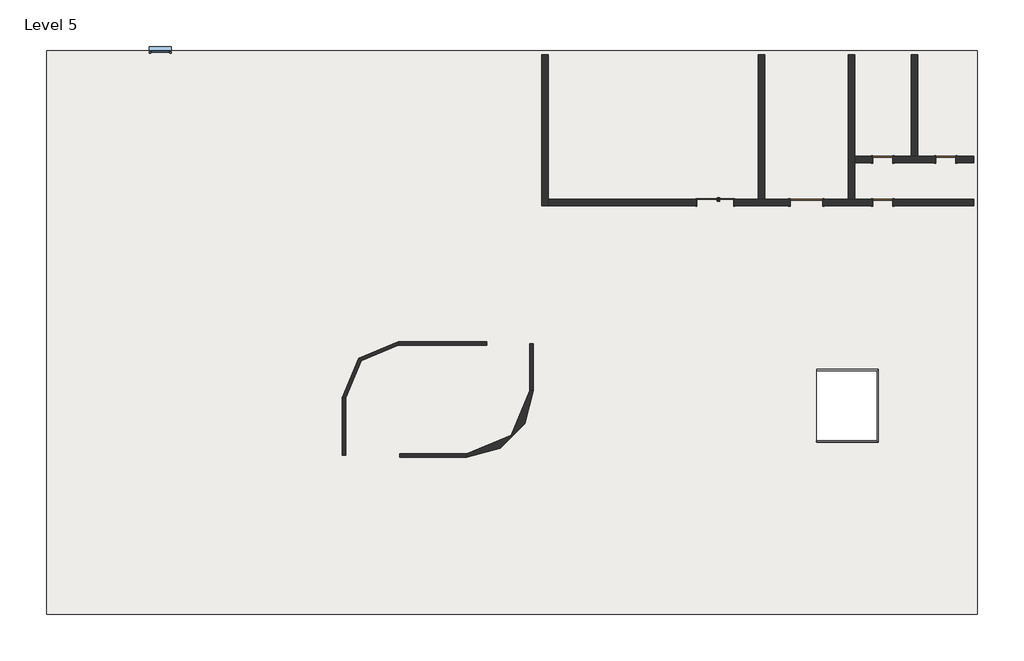
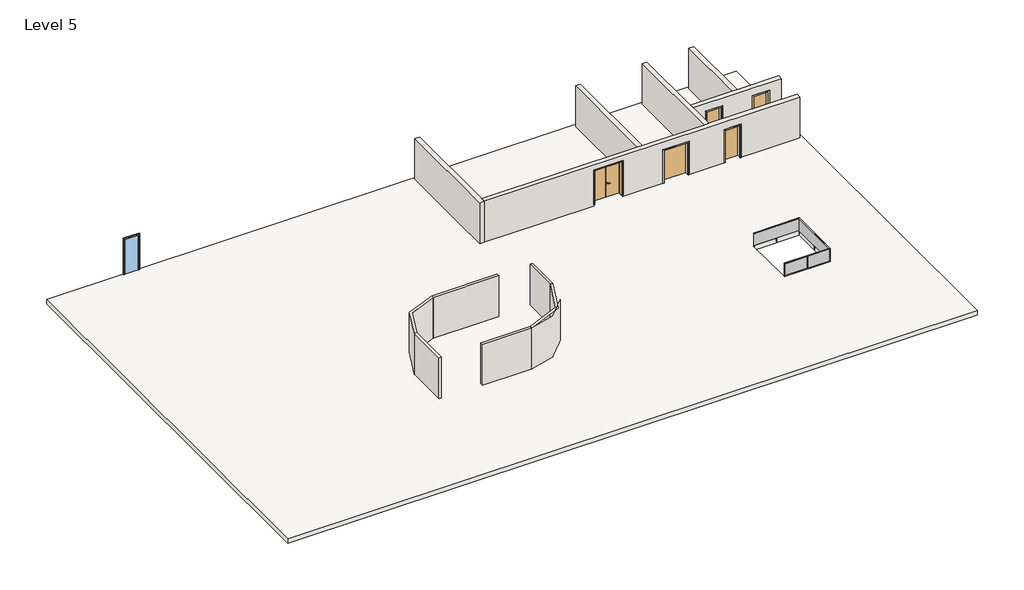
# One storey: 12 walls, 5 doors, 1 railing, 1 slab, 1 window.
"""IFC4 building model written with IfcOpenShell, lengths in millimetres."""

import ifcopenshell
import ifcopenshell.guid

model = None  # the IFC model being written
_history = None  # IfcOwnerHistory: only IFC2X3 demands one
_inside = {}  # id of a spatial element -> (the spatial element, [elements in it])
_under = {}  # id of a project, library or spatial element -> (it, [spatial elements below it])
_declared = {}  # id of a project -> (the project, [libraries it declares])
_typed = {}  # id of a type object -> (the type object, [elements of that type])
_made_of = {}  # id of a material, layer set ... -> (it, [elements and type objects made of it])


def new_model(schema):
    """Start an empty IFC model of exactly this schema.

    Asked for "IFC4X3", IfcOpenShell would pick the latest addendum, in which some entities
    have other attributes; the version numbers below select the first issue.
    IFC2X3 requires an IfcOwnerHistory on every rooted entity: one is made here for all.
    """
    global model, _history
    if schema == "IFC4X3":
        model = ifcopenshell.file(schema_version=(4, 3, 0, 0))
    else:
        model = ifcopenshell.file(schema=schema)
    _inside.clear()
    _under.clear()
    _declared.clear()
    _typed.clear()
    _made_of.clear()
    _history = None
    if model.schema == "IFC2X3":
        org = make("IfcOrganization", Name="unknown")
        user = make(
            "IfcPersonAndOrganization",
            ThePerson=make("IfcPerson", FamilyName="unknown"),
            TheOrganization=org,
        )
        app = make(
            "IfcApplication",
            ApplicationDeveloper=org,
            Version="unknown",
            ApplicationFullName="unknown",
            ApplicationIdentifier="unknown",
        )
        _history = make(
            "IfcOwnerHistory",
            OwningUser=user,
            OwningApplication=app,
            ChangeAction="ADDED",
            CreationDate=0,
        )
    return model


def make(cls, **values):
    """One entity of the class cls with the attributes given. An attribute that is None is left unset."""
    return model.create_entity(
        cls, **{name: value for name, value in values.items() if value is not None}
    )


def rooted(cls, **values):
    """An entity with a GlobalId (a new one), such as an element, a storey or a relation."""
    return make(cls, GlobalId=ifcopenshell.guid.new(), OwnerHistory=_history, **values)


def si_unit(unit_type, name, prefix=None):
    """IfcSIUnit, for example si_unit("LENGTHUNIT", "METRE", prefix="MILLI")."""
    return make("IfcSIUnit", UnitType=unit_type, Prefix=prefix, Name=name)


def assignment(units):
    """IfcUnitAssignment: the units of a project."""
    return None if units is None else make("IfcUnitAssignment", Units=units)


def point(xyz):
    """IfcCartesianPoint."""
    return None if xyz is None else make("IfcCartesianPoint", Coordinates=xyz)


def direction(xyz):
    """IfcDirection."""
    return None if xyz is None else make("IfcDirection", DirectionRatios=xyz)


def frame(location, z_axis=None, x_axis=None):
    """IfcAxis2Placement3D, a coordinate frame: its origin and axes. An axis left out is left unset."""
    return make(
        "IfcAxis2Placement3D",
        Location=point(location),
        Axis=direction(z_axis),
        RefDirection=direction(x_axis),
    )


def frame_2d(location, x_axis=None):
    """IfcAxis2Placement2D, a coordinate frame in the plane: its origin and x axis."""
    return make(
        "IfcAxis2Placement2D", Location=point(location), RefDirection=direction(x_axis)
    )


def origin():
    """The frame at (0, 0, 0) with its axes left unset."""
    return frame((0.0, 0.0, 0.0))


def origin_with_axes():
    """The frame at (0, 0, 0) with the z axis (0, 0, 1) and the x axis (1, 0, 0) written out."""
    return frame((0.0, 0.0, 0.0), z_axis=(0.0, 0.0, 1.0), x_axis=(1.0, 0.0, 0.0))


def place(relative_to, where):
    """IfcLocalPlacement: puts the frame where relative to a parent placement (None: the world)."""
    return make(
        "IfcLocalPlacement", PlacementRelTo=relative_to, RelativePlacement=where
    )


def context(
    kind, dimensions, precision=None, world=None, true_north=None, identifier=None
):
    """IfcGeometricRepresentationContext, for example the 3D "Model" context."""
    return make(
        "IfcGeometricRepresentationContext",
        ContextIdentifier=identifier,
        ContextType=kind,
        CoordinateSpaceDimension=dimensions,
        Precision=precision,
        WorldCoordinateSystem=world,
        TrueNorth=true_north,
    )


def project(units=None, contexts=None):
    """IfcProject with its units and contexts."""
    return rooted(
        "IfcProject",
        Name="project",
        RepresentationContexts=contexts,
        UnitsInContext=assignment(units),
    )


def spatial(cls, under=None, at=None, **own):
    """A site, building, storey or space (cls), placed at a placement, below another one or the project."""
    s = rooted(cls, ObjectPlacement=at, **own)
    if under is not None:
        _under.setdefault(under.id(), (under, []))[1].append(s)
    return s


def polyline(points):
    """IfcPolyline through the points."""
    return make("IfcPolyline", Points=[point(p) for p in points])


def circle_curve(where, radius):
    """IfcCircle in the frame where."""
    return make("IfcCircle", Position=where, Radius=radius)


def ellipse_curve(where, semi_axis1, semi_axis2):
    """IfcEllipse in the frame where."""
    return make(
        "IfcEllipse", Position=where, SemiAxis1=semi_axis1, SemiAxis2=semi_axis2
    )


def trimmed(basis, trim1, trim2, sense, master):
    """IfcTrimmedCurve: the piece of a basis curve between two trims."""
    return make(
        "IfcTrimmedCurve",
        BasisCurve=basis,
        Trim1=trim1,
        Trim2=trim2,
        SenseAgreement=sense,
        MasterRepresentation=master,
    )


def segment(curve, same_sense, transition):
    """IfcCompositeCurveSegment."""
    return make(
        "IfcCompositeCurveSegment",
        Transition=transition,
        SameSense=same_sense,
        ParentCurve=curve,
    )


def composite_curve(segments, self_intersect=None):
    """IfcCompositeCurve: segments joined end to end."""
    return make("IfcCompositeCurve", Segments=segments, SelfIntersect=self_intersect)


def outline(outer, holes=None, kind="AREA"):
    """IfcArbitraryClosedProfileDef: a profile drawn as a closed curve; with holes, ...WithVoids."""
    if holes is None:
        return make("IfcArbitraryClosedProfileDef", ProfileType=kind, OuterCurve=outer)
    return make(
        "IfcArbitraryProfileDefWithVoids",
        ProfileType=kind,
        OuterCurve=outer,
        InnerCurves=holes,
    )


def extrude(swept, where, along, depth):
    """IfcExtrudedAreaSolid: the profile swept, set in the frame where, extruded along a direction by depth."""
    return make(
        "IfcExtrudedAreaSolid",
        SweptArea=swept,
        Position=where,
        ExtrudedDirection=direction(along),
        Depth=depth,
    )


def faces_of(points, faces, orient=None, outer=None):
    """IfcFace entities. A face is a list of loops; a loop is a list of indices into points, from 0.

    orient and outer hold one flag for each loop. By default every Orientation is true, the
    first loop of a face is its IfcFaceOuterBound and the others are IfcFaceBound.
    """
    made = []
    for i, loops in enumerate(faces):
        bounds = []
        for j, loop in enumerate(loops):
            is_outer = j == 0 if outer is None else outer[i][j]
            bounds.append(
                make(
                    "IfcFaceOuterBound" if is_outer else "IfcFaceBound",
                    Bound=make("IfcPolyLoop", Polygon=[points[k] for k in loop]),
                    Orientation=True if orient is None else orient[i][j],
                )
            )
        made.append(make("IfcFace", Bounds=bounds))
    return made


def faceted_brep(points, faces, orient=None, outer=None, voids=None):
    """IfcFacetedBrep: a solid bounded by flat faces; with voids (closed shells), ...WithVoids."""
    shared = [point(p) for p in points]
    hull = make("IfcClosedShell", CfsFaces=faces_of(shared, faces, orient, outer))
    if voids is None:
        return make("IfcFacetedBrep", Outer=hull)
    return make(
        "IfcFacetedBrepWithVoids",
        Outer=hull,
        Voids=[
            make(cls, CfsFaces=faces_of(shared, fs, o, b)) for cls, fs, o, b in voids
        ],
    )


def shape(context_of_items, identifier, shape_type, items):
    """IfcShapeRepresentation: the items that make up one representation, for example the "Body"."""
    return make(
        "IfcShapeRepresentation",
        ContextOfItems=context_of_items,
        RepresentationIdentifier=identifier,
        RepresentationType=shape_type,
        Items=items,
    )


def source(mapping_origin, context_of_items, identifier, shape_type, items):
    """IfcRepresentationMap: a shape defined once, which mapped items show again and again."""
    return make(
        "IfcRepresentationMap",
        MappingOrigin=mapping_origin,
        MappedRepresentation=shape(context_of_items, identifier, shape_type, items),
    )


def transform(
    local_origin,
    x_axis=None,
    y_axis=None,
    z_axis=None,
    scale=None,
    scale2=None,
    scale3=None,
    uniform=True,
):
    """IfcCartesianTransformationOperator3D, or its non-uniform kind. x_axis, y_axis, z_axis: its Axis1, 2, 3."""
    if uniform:
        return make(
            "IfcCartesianTransformationOperator3D",
            Axis1=direction(x_axis),
            Axis2=direction(y_axis),
            LocalOrigin=point(local_origin),
            Scale=scale,
            Axis3=direction(z_axis),
        )
    return make(
        "IfcCartesianTransformationOperator3DnonUniform",
        Axis1=direction(x_axis),
        Axis2=direction(y_axis),
        LocalOrigin=point(local_origin),
        Scale=scale,
        Axis3=direction(z_axis),
        Scale2=scale2,
        Scale3=scale3,
    )


def mapped(mapping_source, mapping_target):
    """IfcMappedItem: shows the shape of a source again, moved by a transform."""
    return make(
        "IfcMappedItem", MappingSource=mapping_source, MappingTarget=mapping_target
    )


def made_of(thing, what):
    """Note that an element or type object is made of a material, layer set ...; save() writes the relation."""
    if what is not None:
        _made_of.setdefault(what.id(), (what, []))[1].append(thing)
    return thing


def element(
    cls,
    number,
    at=None,
    inside=None,
    cuts=None,
    type_object=None,
    material=None,
    context=None,
    identifier="Body",
    shape_type=None,
    held_by="IfcProductDefinitionShape",
    body=None,
    shapes=None,
    **own,
):
    """One element of the class cls, such as IfcWall. Its Tag is "e" and its number.

    at: its placement. inside: the storey or other place that contains it. cuts: it is an
    opening in that element (IfcRelVoidsElement). A single representation is given by context,
    identifier, shape_type and body (its items); several are given by shapes. held_by: the class
    of the entity that holds the representations. save() writes the other relations.
    """
    e = rooted(cls, Tag="e%d" % number, ObjectPlacement=at, **own)
    if body is not None:
        shapes = [shape(context, identifier, shape_type, body)]
    if shapes is not None:
        e.Representation = make(held_by, Representations=shapes)
    if inside is not None:
        _inside.setdefault(inside.id(), (inside, []))[1].append(e)
    if cuts is not None:
        rooted(
            "IfcRelVoidsElement", RelatingBuildingElement=cuts, RelatedOpeningElement=e
        )
    if type_object is not None:
        _typed.setdefault(type_object.id(), (type_object, []))[1].append(e)
    return made_of(e, material)


def aggregate(whole, parts):
    """IfcRelAggregates: a whole, such as a stair, and the parts it consists of."""
    return rooted("IfcRelAggregates", RelatingObject=whole, RelatedObjects=parts)


def save(model, path):
    """Write the relations noted so far, then the file.

    IfcRelAggregates (storeys below a building ...), IfcRelContainedInSpatialStructure (elements
    in a storey), IfcRelDefinesByType, IfcRelAssociatesMaterial and IfcRelDeclares: one each for
    every whole, place, type object, material and project.
    """
    for whole, parts in _under.values():
        aggregate(whole, parts)
    for where, things in _inside.values():
        rooted(
            "IfcRelContainedInSpatialStructure",
            RelatedElements=things,
            RelatingStructure=where,
        )
    for kind, things in _typed.values():
        rooted("IfcRelDefinesByType", RelatedObjects=things, RelatingType=kind)
    for what, things in _made_of.values():
        rooted("IfcRelAssociatesMaterial", RelatedObjects=things, RelatingMaterial=what)
    for by, libraries in _declared.values():
        rooted("IfcRelDeclares", RelatingContext=by, RelatedDefinitions=libraries)
    model.write(path)


def plane_surface(at):
    """IfcPlane: the flat surface through the origin of the frame at, square to its z axis."""
    return make("IfcPlane", Position=at)


def cylinder_surface(at, radius):
    """IfcCylindricalSurface: all points at the distance radius from the z axis of the frame at."""
    return make("IfcCylindricalSurface", Position=at, Radius=radius)


def advanced_brep(points, edges, surfaces, faces):
    """IfcAdvancedBrep: a solid bounded by faces that lie on surfaces and meet in shared edges.

    An edge is (start, end): straight between two places in points (the first is 0);
    or (start, end, curve); or (start, end, curve, False) where it runs against its curve.
    A face is (place in surfaces, loops), or (place, loops, False) where it looks against
    its surface's normal. A loop lists edges by number (the first is 1), with a minus sign
    where the edge is run from its end to its start. The first loop is the outer one.
    """
    corners = [point(p) for p in points]
    vertices = [make("IfcVertexPoint", VertexGeometry=c) for c in corners]
    made = []
    for start, end, *more in edges:
        made.append(
            make(
                "IfcEdgeCurve",
                EdgeStart=vertices[start],
                EdgeEnd=vertices[end],
                EdgeGeometry=more[0] if more else make("IfcPolyline", Points=[corners[start], corners[end]]),
                SameSense=more[1] if len(more) > 1 else True,
            )
        )
    hull = []
    for where, loops, *sense in faces:
        bounds = []
        for j, loop in enumerate(loops):
            ring = [make("IfcOrientedEdge", EdgeElement=made[abs(k) - 1], Orientation=k > 0) for k in loop]
            bounds.append(
                make(
                    "IfcFaceOuterBound" if j == 0 else "IfcFaceBound",
                    Bound=make("IfcEdgeLoop", EdgeList=ring),
                    Orientation=True,
                )
            )
        hull.append(make("IfcAdvancedFace", Bounds=bounds, FaceSurface=surfaces[where], SameSense=sense[0] if sense else True))
    return make("IfcAdvancedBrep", Outer=make("IfcClosedShell", CfsFaces=hull))


def door_double_flush_variable_door_double_flush_variable_ac6c3b87(model_context):
    return source(origin(), model_context, "Body", "SolidModel", [
        advanced_brep(
        [(90.0, 139.4346141, 1000.0), (110.0, 139.4346141, 1000.0), (90.0, 69.4346141, 1000.0), (110.0, 89.4346141, 1000.0), (220.0, 69.4346141, 1000.0), (220.0, 89.4346141, 1000.0)],
        [
            (0, 1, circle_curve(frame((100.0, 139.4346141, 1000.0), z_axis=(0.0, 1.0, 0.0), x_axis=(1.0, 0.0, 0.0)), 10.0)),
            (1, 0, circle_curve(frame((100.0, 139.4346141, 1000.0), z_axis=(0.0, 1.0, 0.0), x_axis=(1.0, 0.0, 0.0)), 10.0)),
            (0, 2),
            (2, 3, ellipse_curve(frame((100.0, 79.4346141, 1000.0), z_axis=(-0.7071067811865385, 0.7071067811865565, 0.0), x_axis=(0.7071067811865563, 0.7071067811865386, 0.0)), 14.1421356, 10.0)),
            (3, 1),
            (3, 2, ellipse_curve(frame((100.0, 79.4346141, 1000.0), z_axis=(-0.7071067811865385, 0.7071067811865565, 0.0), x_axis=(0.7071067811865563, 0.7071067811865386, 0.0)), 14.1421356, 10.0)),
            (4, 5, circle_curve(frame((220.0, 79.4346141, 1000.0), z_axis=(1.0, 0.0, 0.0), x_axis=(0.0, 1.0, 0.0)), 10.0)),
            (5, 4, circle_curve(frame((220.0, 79.4346141, 1000.0), z_axis=(1.0, 0.0, 0.0), x_axis=(0.0, 1.0, 0.0)), 10.0)),
            (2, 4),
            (5, 3),
        ],
        [
            plane_surface(frame((100.0, 139.4346141, -287.7526403), z_axis=(0.0, 1.0, 0.0), x_axis=(0.0, 0.0, 1.0))),
            cylinder_surface(frame((100.0, 139.4346141, 1000.0), z_axis=(0.0, 1.0, 0.0), x_axis=(1.0, 0.0, 0.0)), 10.0),
            plane_surface(frame((220.0, 79.4346141, -287.7526403), z_axis=(1.0, 0.0, 0.0), x_axis=(0.0, 0.0, 1.0))),
            cylinder_surface(frame((100.0, 79.4346141, 1000.0), z_axis=(-1.0, 0.0, 0.0), x_axis=(0.0, 1.0, 0.0)), 10.0),
        ],
        [
            (0, [[1, 2]]),
            (1, [[-1, 3, 4, 5]]),
            (1, [[-2, -5, 6, -3]]),
            (2, [[7, 8]]),
            (3, [[-4, 9, -8, 10]]),
            (3, [[-6, -10, -7, -9]]),
        ],
    ),
        advanced_brep(
        [(110.0, 199.4346141, 1000.0), (90.0, 199.4346141, 1000.0), (110.0, 229.4346141, 1000.0), (90.0, 249.4346141, 1000.0), (220.0, 229.4346141, 1000.0), (220.0, 249.4346141, 1000.0)],
        [
            (0, 1, circle_curve(frame((100.0, 199.4346141, 1000.0), z_axis=(0.0, -1.0, 0.0), x_axis=(-1.0, 0.0, 0.0)), 10.0)),
            (1, 0, circle_curve(frame((100.0, 199.4346141, 1000.0), z_axis=(0.0, -1.0, 0.0), x_axis=(-1.0, 0.0, 0.0)), 10.0)),
            (0, 2),
            (2, 3, ellipse_curve(frame((100.0, 239.4346141, 1000.0), z_axis=(-0.7071067811865475, -0.7071067811865475, 0.0), x_axis=(0.7071067811865474, -0.7071067811865476, 0.0)), 14.1421356, 10.0)),
            (3, 1),
            (3, 2, ellipse_curve(frame((100.0, 239.4346141, 1000.0), z_axis=(-0.7071067811865475, -0.7071067811865475, 0.0), x_axis=(0.7071067811865474, -0.7071067811865476, 0.0)), 14.1421356, 10.0)),
            (4, 5, circle_curve(frame((220.0, 239.4346141, 1000.0), z_axis=(1.0, 0.0, 0.0), x_axis=(0.0, 1.0, 0.0)), 10.0)),
            (5, 4, circle_curve(frame((220.0, 239.4346141, 1000.0), z_axis=(1.0, 0.0, 0.0), x_axis=(0.0, 1.0, 0.0)), 10.0)),
            (2, 4),
            (5, 3),
        ],
        [
            plane_surface(frame((100.0, 199.4346141, -287.7526403), z_axis=(0.0, -1.0, 0.0), x_axis=(0.0, 0.0, 1.0))),
            cylinder_surface(frame((100.0, 199.4346141, 1000.0), z_axis=(0.0, -1.0, 0.0), x_axis=(-1.0, 0.0, 0.0)), 10.0),
            plane_surface(frame((220.0, 239.4346141, -287.7526403), z_axis=(1.0, 0.0, 0.0), x_axis=(0.0, 0.0, 1.0))),
            cylinder_surface(frame((100.0, 239.4346141, 1000.0), z_axis=(-1.0, 0.0, 0.0), x_axis=(0.0, 1.0, 0.0)), 10.0),
        ],
        [
            (0, [[1, 2]]),
            (1, [[-1, 3, 4, 5]]),
            (1, [[-2, -5, 6, -3]]),
            (2, [[7, 8]]),
            (3, [[-4, 9, -8, 10]]),
            (3, [[-6, -10, -7, -9]]),
        ],
    ),
        extrude(outline(composite_curve([segment(trimmed(circle_curve(frame_2d((1000.0, 100.0)), 20.0), [point((1000.0, 80.0))], [point((1000.0, 120.0))], False, "CARTESIAN"), True, "CONTINUOUS"), segment(trimmed(circle_curve(frame_2d((1000.0, 100.0)), 20.0), [point((1000.0, 120.0))], [point((1000.0, 80.0))], False, "CARTESIAN"), True, "CONTINUOUS")], self_intersect=False)), frame((0.0, 129.4346141, 0.0), z_axis=(0.0, 1.0, 0.0), x_axis=(0.0, 0.0, 1.0)), (0.0, 0.0, 1.0), 10.0),
        extrude(outline(composite_curve([segment(trimmed(circle_curve(frame_2d((1000.0, 100.0)), 20.0), [point((1000.0, 80.0))], [point((1000.0, 120.0))], False, "CARTESIAN"), True, "CONTINUOUS"), segment(trimmed(circle_curve(frame_2d((1000.0, 100.0)), 20.0), [point((1000.0, 120.0))], [point((1000.0, 80.0))], False, "CARTESIAN"), True, "CONTINUOUS")], self_intersect=False)), frame((0.0, 189.4346141, 0.0), z_axis=(0.0, 1.0, 0.0), x_axis=(0.0, 0.0, 1.0)), (0.0, 0.0, 1.0), 10.0),
        extrude(outline(polyline([(0.0, 164.4346141), (-871.25, 164.4346141), (-871.25, 189.4346141), (0.0, 189.4346141), (0.0, 164.4346141)])), frame((0.0, 0.0, 100.0), z_axis=(0.0, 0.0, 1.0), x_axis=(1.0, 0.0, 0.0)), (0.0, 0.0, 1.0), 2250.0),
        extrude(outline(polyline([(871.25, 164.4346141), (0.0, 164.4346141), (0.0, 189.4346141), (871.25, 189.4346141), (871.25, 164.4346141)])), frame((0.0, 0.0, 100.0), z_axis=(0.0, 0.0, 1.0), x_axis=(1.0, 0.0, 0.0)), (0.0, 0.0, 1.0), 2250.0),
        faceted_brep([(905.75, -150.5653859, 100.0), (856.25, -150.5653859, 100.0), (856.25, 164.4346141, 100.0), (871.25, 164.4346141, 100.0), (871.25, 189.4346141, 100.0), (905.75, 189.4346141, 100.0), (905.75, 164.4346141, 100.0), (900.75, 164.4346141, 100.0), (900.75, 184.4346141, 100.0), (876.25, 184.4346141, 100.0), (876.25, 159.4346141, 100.0), (861.25, 159.4346141, 100.0), (861.25, -145.5653859, 100.0), (900.75, -145.5653859, 100.0), (900.75, -135.5653859, 100.0), (905.75, -135.5653859, 100.0), (905.75, -150.5653859, 2384.5), (-905.75, -150.5653859, 2384.5), (-905.75, -150.5653859, 100.0), (-856.25, -150.5653859, 100.0), (-856.25, -150.5653859, 2335.0), (856.25, -150.5653859, 2335.0), (856.25, 164.4346141, 2335.0), (-856.25, 164.4346141, 2335.0), (-856.25, 164.4346141, 100.0), (-871.25, 164.4346141, 100.0), (-871.25, 164.4346141, 2350.0), (871.25, 164.4346141, 2350.0), (871.25, 189.4346141, 2350.0), (-871.25, 189.4346141, 2350.0), (-871.25, 189.4346141, 100.0), (-905.75, 189.4346141, 100.0), (-905.75, 189.4346141, 2384.5), (905.75, 189.4346141, 2384.5), (905.75, 164.4346141, 2384.5), (-905.75, 164.4346141, 2384.5), (-905.75, 164.4346141, 100.0), (-900.75, 164.4346141, 100.0), (-900.75, 164.4346141, 2379.5), (900.75, 164.4346141, 2379.5), (900.75, 184.4346141, 2379.5), (-900.75, 184.4346141, 2379.5), (-900.75, 184.4346141, 100.0), (-876.25, 184.4346141, 100.0), (-876.25, 184.4346141, 2355.0), (876.25, 184.4346141, 2355.0), (876.25, 159.4346141, 2355.0), (-876.25, 159.4346141, 2355.0), (-876.25, 159.4346141, 100.0), (-861.25, 159.4346141, 100.0), (-861.25, 159.4346141, 2340.0), (861.25, 159.4346141, 2340.0), (861.25, -145.5653859, 2340.0), (-861.25, -145.5653859, 2340.0), (-861.25, -145.5653859, 100.0), (-900.75, -145.5653859, 100.0), (-900.75, -145.5653859, 2379.5), (900.75, -145.5653859, 2379.5), (900.75, -135.5653859, 2379.5), (-900.75, -135.5653859, 2379.5), (-900.75, -135.5653859, 100.0), (-905.75, -135.5653859, 100.0), (-905.75, -135.5653859, 2384.5), (905.75, -135.5653859, 2384.5)], [[[0, 1, 2, 3, 4, 5, 6, 7, 8, 9, 10, 11, 12, 13, 14, 15]], [[1, 0, 16, 17, 18, 19, 20, 21]], [[2, 1, 21, 22]], [[3, 2, 22, 23, 24, 25, 26, 27]], [[4, 3, 27, 28]], [[5, 4, 28, 29, 30, 31, 32, 33]], [[6, 5, 33, 34]], [[7, 6, 34, 35, 36, 37, 38, 39]], [[8, 7, 39, 40]], [[9, 8, 40, 41, 42, 43, 44, 45]], [[10, 9, 45, 46]], [[11, 10, 46, 47, 48, 49, 50, 51]], [[12, 11, 51, 52]], [[13, 12, 52, 53, 54, 55, 56, 57]], [[14, 13, 57, 58]], [[15, 14, 58, 59, 60, 61, 62, 63]], [[0, 15, 63, 16]], [[17, 62, 61, 18]], [[18, 61, 60, 55, 54, 49, 48, 43, 42, 37, 36, 31, 30, 25, 24, 19]], [[23, 20, 19, 24]], [[29, 26, 25, 30]], [[35, 32, 31, 36]], [[41, 38, 37, 42]], [[47, 44, 43, 48]], [[53, 50, 49, 54]], [[59, 56, 55, 60]], [[22, 21, 20, 23]], [[28, 27, 26, 29]], [[34, 33, 32, 35]], [[40, 39, 38, 41]], [[46, 45, 44, 47]], [[52, 51, 50, 53]], [[58, 57, 56, 59]], [[16, 63, 62, 17]]]),
    ])


def m_single_flush_0915_x_2134mm_1c84716f(model_context):
    return source(origin(), model_context, "Body", "SweptSolid", [
        extrude(outline(polyline([(2210.0, -533.5), (0.0, -533.5), (0.0, -457.5), (2134.0, -457.5), (2134.0, 457.5), (0.0, 457.5), (0.0, 533.5), (2210.0, 533.5), (2210.0, -533.5)])), frame((0.0, -175.0, 0.0), z_axis=(0.0, 1.0, 0.0), x_axis=(0.0, 0.0, 1.0)), (0.0, 0.0, 1.0), 25.0),
        extrude(outline(polyline([(2210.0, 533.5), (2210.0, -533.5), (0.0, -533.5), (0.0, -457.5), (2134.0, -457.5), (2134.0, 457.5), (0.0, 457.5), (0.0, 533.5), (2210.0, 533.5)])), frame((0.0, 150.0, 0.0), z_axis=(0.0, 1.0, 0.0), x_axis=(0.0, 0.0, 1.0)), (0.0, 0.0, 1.0), 25.0),
        extrude(outline(polyline([(457.5, -99.0), (457.5, -150.0), (-457.5, -150.0), (-457.5, -99.0), (457.5, -99.0)])), origin_with_axes(), (0.0, 0.0, 1.0), 2134.0),
    ])


def m_single_flush_1500_x_2134mm_2_edebd810(model_context):
    return source(origin(), model_context, "Body", "SweptSolid", [
        extrude(outline(polyline([(2210.0, -826.0), (0.0, -826.0), (0.0, -750.0), (2134.0, -750.0), (2134.0, 750.0), (0.0, 750.0), (0.0, 826.0), (2210.0, 826.0), (2210.0, -826.0)])), frame((0.0, -175.0, 0.0), z_axis=(0.0, 1.0, 0.0), x_axis=(0.0, 0.0, 1.0)), (0.0, 0.0, 1.0), 25.0),
        extrude(outline(polyline([(2210.0, 826.0), (2210.0, -826.0), (0.0, -826.0), (0.0, -750.0), (2134.0, -750.0), (2134.0, 750.0), (0.0, 750.0), (0.0, 826.0), (2210.0, 826.0)])), frame((0.0, 150.0, 0.0), z_axis=(0.0, 1.0, 0.0), x_axis=(0.0, 0.0, 1.0)), (0.0, 0.0, 1.0), 25.0),
        extrude(outline(polyline([(750.0, -99.0), (750.0, -150.0), (-750.0, -150.0), (-750.0, -99.0), (750.0, -99.0)])), origin_with_axes(), (0.0, 0.0, 1.0), 2134.0),
    ])


def glas_mpk_389492d2(model_context):
    return source(origin(), model_context, "Body", "SolidModel", [
        faceted_brep([(28820.4268037, 1294.9571597, 12843.2628643), (28820.4268037, 1244.9571597, 12843.2628643), (28820.4268037, 1244.9571597, 12856.7371357), (28820.4268037, 1294.9571597, 12856.7371357), (31660.4268037, 1294.9571597, 12843.2628643), (31610.4268037, 1244.9571597, 12843.2628643), (31610.4268037, 1244.9571597, 12856.7371357), (31660.4268037, 1294.9571597, 12856.7371357), (31660.4268037, -2045.7721864, 12843.2628643), (31610.4268037, -1995.7721864, 12843.2628643), (31610.4268037, -1995.7721864, 12856.7371357), (31660.4268037, -2045.7721864, 12856.7371357), (28820.4268037, -2045.7721864, 12843.2628643), (28820.4268037, -2045.7721864, 12856.7371357), (28820.4268037, -1995.7721864, 12856.7371357), (28820.4268037, -1995.7721864, 12843.2628643)], [[[0, 1, 2, 3]], [[1, 0, 4, 5]], [[2, 1, 5, 6]], [[3, 2, 6, 7]], [[0, 3, 7, 4]], [[5, 4, 8, 9]], [[6, 5, 9, 10]], [[7, 6, 10, 11]], [[4, 7, 11, 8]], [[12, 13, 14, 15]], [[9, 8, 12, 15]], [[10, 9, 15, 14]], [[11, 10, 14, 13]], [[8, 11, 13, 12]]]),
        faceted_brep([(28820.4268037, 1254.9571597, 12842.8769824), (28820.4268037, 1269.1492837, 12842.8769824), (28820.4268037, 1269.1492837, 12042.8769824), (28820.4268037, 1254.9571597, 12042.8769824), (31620.4268037, 1254.9571597, 12842.8769824), (31634.6189277, 1269.1492837, 12842.8769824), (31634.6189277, 1269.1492837, 12042.8769824), (31620.4268037, 1254.9571597, 12042.8769824), (31620.4268037, -2005.7721864, 12842.8769824), (31634.6189277, -2019.9643104, 12842.8769824), (31634.6189277, -2019.9643104, 12042.8769824), (31620.4268037, -2005.7721864, 12042.8769824), (28820.4268037, -2005.7721864, 12842.8769824), (28820.4268037, -2005.7721864, 12042.8769824), (28820.4268037, -2019.9643104, 12042.8769824), (28820.4268037, -2019.9643104, 12842.8769824)], [[[0, 1, 2, 3]], [[1, 0, 4, 5]], [[2, 1, 5, 6]], [[3, 2, 6, 7]], [[0, 3, 7, 4]], [[5, 4, 8, 9]], [[6, 5, 9, 10]], [[7, 6, 10, 11]], [[4, 7, 11, 8]], [[12, 13, 14, 15]], [[9, 8, 12, 15]], [[10, 9, 15, 14]], [[11, 10, 14, 13]], [[8, 11, 13, 12]]]),
        extrude(outline(polyline([(30251.6768037, -2020.7721864), (30251.6768037, -2045.7721864), (30226.6768037, -2045.7721864), (30226.6768037, -2020.7721864), (30251.6768037, -2020.7721864)])), frame((0.0, 0.0, 11800.0), z_axis=(0.0, 0.0, 1.0), x_axis=(1.0, 0.0, 0.0)), (0.0, 0.0, 1.0), 1043.2628643),
        extrude(outline(polyline([(31635.4268037, -362.9075133), (31660.4268037, -362.9075133), (31660.4268037, -387.9075133), (31635.4268037, -387.9075133), (31635.4268037, -362.9075133)])), frame((0.0, 0.0, 11800.0), z_axis=(0.0, 0.0, 1.0), x_axis=(1.0, 0.0, 0.0)), (0.0, 0.0, 1.0), 1043.2628643),
        extrude(outline(polyline([(30226.6768037, 1269.9571597), (30226.6768037, 1294.9571597), (30251.6768037, 1294.9571597), (30251.6768037, 1269.9571597), (30226.6768037, 1269.9571597)])), frame((0.0, 0.0, 11800.0), z_axis=(0.0, 0.0, 1.0), x_axis=(1.0, 0.0, 0.0)), (0.0, 0.0, 1.0), 1043.2628643),
        extrude(outline(polyline([(31635.4268037, -2030.7721864), (31660.4268037, -2030.7721864), (31660.4268037, -2055.7721864), (31635.4268037, -2055.7721864), (31635.4268037, -2030.7721864)])), frame((0.0, 0.0, 11800.0), z_axis=(0.0, 0.0, 1.0), x_axis=(1.0, 0.0, 0.0)), (0.0, 0.0, 1.0), 1043.2628643),
        extrude(outline(polyline([(31645.4268037, 1269.9571597), (31645.4268037, 1294.9571597), (31670.4268037, 1294.9571597), (31670.4268037, 1269.9571597), (31645.4268037, 1269.9571597)])), frame((0.0, 0.0, 11800.0), z_axis=(0.0, 0.0, 1.0), x_axis=(1.0, 0.0, 0.0)), (0.0, 0.0, 1.0), 1043.2628643),
        extrude(outline(polyline([(28832.9268037, -2020.7721864), (28832.9268037, -2045.7721864), (28807.9268037, -2045.7721864), (28807.9268037, -2020.7721864), (28832.9268037, -2020.7721864)])), frame((0.0, 0.0, 11800.0), z_axis=(0.0, 0.0, 1.0), x_axis=(1.0, 0.0, 0.0)), (0.0, 0.0, 1.0), 1043.2628643),
        extrude(outline(polyline([(28820.4268037, 1269.9571597), (28820.4268037, 1294.9571597), (28845.4268037, 1294.9571597), (28845.4268037, 1269.9571597), (28820.4268037, 1269.9571597)])), frame((0.0, 0.0, 11800.0), z_axis=(0.0, 0.0, 1.0), x_axis=(1.0, 0.0, 0.0)), (0.0, 0.0, 1.0), 1043.2628643),
    ])


def window_variable_standard_5cf830ff(model_context):
    return source(origin(), model_context, "Body", "SolidModel", [
        extrude(outline(polyline([(9000.0, 500.0), (9000.0, -500.0), (1000.0, -500.0), (1000.0, 500.0), (9000.0, 500.0)]), holes=[polyline([(8920.0, 440.0), (1080.0, 440.0), (1080.0, -440.0), (8920.0, -440.0), (8920.0, 440.0)])]), frame((0.0, 35.0, 0.0), z_axis=(0.0, 1.0, 0.0), x_axis=(0.0, 0.0, 1.0)), (0.0, 0.0, 1.0), 60.0),
        faceted_brep([(470.0, 35.0, 8950.0), (470.0, 5.0, 8950.0), (470.0, 5.0, 1050.0), (470.0, 35.0, 1050.0), (-470.0, 5.0, 8950.0), (-470.0, 5.0, 1050.0), (410.0, 5.0, 1110.0), (-410.0, 5.0, 1110.0), (-410.0, 5.0, 8890.0), (410.0, 5.0, 8890.0), (-470.0, 35.0, 1050.0), (-470.0, 35.0, 8950.0), (440.0, 35.0, 8920.0), (-440.0, 35.0, 8920.0), (-440.0, 35.0, 1080.0), (440.0, 35.0, 1080.0), (440.0, 65.0, 8920.0), (440.0, 65.0, 1080.0), (-440.0, 65.0, 1080.0), (-440.0, 65.0, 8920.0), (410.0, 65.0, 8890.0), (-410.0, 65.0, 8890.0), (-410.0, 65.0, 1110.0), (410.0, 65.0, 1110.0)], [[[0, 1, 2, 3]], [[1, 4, 5, 2], [6, 7, 8, 9]], [[3, 2, 5, 10]], [[3, 10, 11, 0], [12, 13, 14, 15]], [[16, 12, 15, 17]], [[17, 15, 14, 18]], [[17, 18, 19, 16], [20, 21, 22, 23]], [[9, 20, 23, 6]], [[6, 23, 22, 7]], [[10, 5, 4, 11]], [[18, 14, 13, 19]], [[7, 22, 21, 8]], [[11, 4, 1, 0]], [[19, 13, 12, 16]], [[8, 21, 20, 9]]]),
        extrude(outline(polyline([(-500.0, -205.0), (-500.0, 35.0), (500.0, 35.0), (500.0, -205.0), (-500.0, -205.0)])), frame((0.0, 0.0, 1005.0), z_axis=(0.0, 0.0, 1.0), x_axis=(1.0, 0.0, 0.0)), (0.0, 0.0, 1.0), 15.0),
        extrude(outline(polyline([(105.0221543, 1020.0), (205.0, 1000.0), (205.0, 990.0), (203.0, 990.0), (203.0, 998.3604634), (104.8240723, 1018.0), (95.0, 1018.0), (95.0, 1020.0), (105.0221543, 1020.0)])), frame((-500.0, 0.0, 0.0), z_axis=(1.0, 0.0, 0.0), x_axis=(0.0, 1.0, 0.0)), (0.0, 0.0, 1.0), 1000.0),
        extrude(outline(polyline([(410.0, 20.0), (-410.0, 20.0), (-410.0, 50.0), (410.0, 50.0), (410.0, 20.0)])), frame((0.0, 0.0, 1110.0), z_axis=(0.0, 0.0, 1.0), x_axis=(1.0, 0.0, 0.0)), (0.0, 0.0, 1.0), 7780.0),
    ])


model = new_model("IFC4")

# Units and contexts
model_context = context("Model", 3, world=origin())
ifc_project = project(units=[si_unit("LENGTHUNIT", "METRE", prefix="MILLI")], contexts=[model_context])

# Site, building, storey
site = spatial("IfcSite", under=ifc_project)
building = spatial("IfcBuilding", under=site)
storey = spatial("IfcBuildingStorey", under=building, Name="Level 5", Elevation=12000.0)

# Doors
placement = place(None, origin())
door_double_flush_variable_door_double_flush_variable_shape = door_double_flush_variable_door_double_flush_variable_ac6c3b87(model_context)
element("IfcDoor", 1, ObjectType="Door Double Flush - Variable : Door Double Flush - Variable", at=placement, inside=storey, context=model_context, shape_type="MappedRepresentation", body=[
    mapped(door_double_flush_variable_door_double_flush_variable_shape, transform((24136.7471367, 8984.3231089, 12000.0), x_axis=(1.0, 0.0, 0.0), y_axis=(0.0, 1.0, 0.0), z_axis=(0.0, 0.0, 1.0))),
])
m_single_flush_0915_x_2134mm_shape = m_single_flush_0915_x_2134mm_1c84716f(model_context)
element("IfcDoor", 2, ObjectType="M_Single-Flush : 0915 x 2134mm", at=placement, inside=storey, context=model_context, shape_type="MappedRepresentation", body=[
    mapped(m_single_flush_0915_x_2134mm_shape, transform((34787.1221367, 10998.757723, 12000.0), x_axis=(-1.0, 0.0, 0.0), y_axis=(0.0, -1.0, 0.0), z_axis=(0.0, 0.0, 1.0))),
])
element("IfcDoor", 3, ObjectType="M_Single-Flush : 0915 x 2134mm", at=placement, inside=storey, context=model_context, shape_type="MappedRepresentation", body=[
    mapped(m_single_flush_0915_x_2134mm_shape, transform((31874.3721367, 10998.757723, 12000.0), x_axis=(-1.0, 0.0, 0.0), y_axis=(0.0, -1.0, 0.0), z_axis=(0.0, 0.0, 1.0))),
])
element("IfcDoor", 4, ObjectType="M_Single-Flush : 0915 x 2134mm", at=placement, inside=storey, context=model_context, shape_type="MappedRepresentation", body=[
    mapped(m_single_flush_0915_x_2134mm_shape, transform((31874.3721367, 8998.757723, 12000.0), x_axis=(-1.0, 0.0, 0.0), y_axis=(0.0, -1.0, 0.0), z_axis=(0.0, 0.0, 1.0))),
])
m_single_flush_1500_x_2134mm_2_shape = m_single_flush_1500_x_2134mm_2_edebd810(model_context)
element("IfcDoor", 5, ObjectType="M_Single-Flush : 1500 x 2134mm 2", at=placement, inside=storey, context=model_context, shape_type="MappedRepresentation", body=[
    mapped(m_single_flush_1500_x_2134mm_2_shape, transform((28342.9971367, 8998.757723, 12000.0), x_axis=(-1.0, 0.0, 0.0), y_axis=(0.0, -1.0, 0.0), z_axis=(0.0, 0.0, 1.0))),
])

# Railing
glas_mpk_shape = glas_mpk_389492d2(model_context)
element("IfcRailing", 6, ObjectType="Glas - MPK", at=placement, inside=storey, context=model_context, shape_type="MappedRepresentation", body=[
    mapped(glas_mpk_shape, transform((0.0, 0.0, 0.0), x_axis=(1.0, 0.0, 0.0), y_axis=(0.0, 1.0, 0.0), z_axis=(0.0, 0.0, 1.0))),
])

# Slab
element("IfcSlab", 7, ObjectType="Generic 300mm", at=placement, inside=storey, context=model_context, shape_type="SweptSolid", body=[
    extrude(outline(polyline([(-6732.0028633, 15998.757723), (36243.4971367, 15998.757723), (36243.4971367, -10001.242277), (-6732.0028633, -10001.242277), (-6732.0028633, 15998.757723)]), holes=[polyline([(31663.0737371, 1305.1195288), (28813.0737371, 1305.1195288), (28813.0737371, -2055.6098174), (31663.0737371, -2055.6098174), (31663.0737371, 1305.1195288)])]), frame((0.0, 0.0, 11700.0), z_axis=(0.0, 0.0, 1.0), x_axis=(1.0, 0.0, 0.0)), (0.0, 0.0, 1.0), 300.0),
])

# Walls
element("IfcWall", 8, ObjectType="Generic - 300mm", at=placement, inside=storey, context=model_context, shape_type="Brep", body=[
    faceted_brep([(16117.9971367, 15823.757723, 12000.0), (16117.9971367, 8848.757723, 12000.0), (16117.9971367, 8848.757723, 14700.0), (16117.9971367, 15823.757723, 14700.0), (16417.9971367, 15823.757723, 12000.0), (16417.9971367, 15823.757723, 14700.0), (16417.9971367, 9148.757723, 14700.0), (16417.9971367, 8848.757723, 14700.0), (16417.9971367, 8848.757723, 12000.0), (16417.9971367, 9148.757723, 12000.0)], [[[0, 1, 2, 3]], [[4, 5, 6, 7, 8, 9]], [[1, 0, 4, 9, 8]], [[3, 2, 7, 6, 5]], [[2, 1, 8, 7]], [[0, 3, 5, 4]]]),
])
element("IfcWall", 9, ObjectType="Generic - 300mm", at=placement, inside=storey, context=model_context, shape_type="SweptSolid", body=[
    extrude(outline(polyline([(26117.9971367, 9148.757723), (26117.9971367, 15823.757723), (26417.9971367, 15823.757723), (26417.9971367, 9148.757723), (26117.9971367, 9148.757723)])), frame((0.0, 0.0, 12000.0), z_axis=(0.0, 0.0, 1.0), x_axis=(1.0, 0.0, 0.0)), (0.0, 0.0, 1.0), 2700.0),
])
element("IfcWall", 10, ObjectType="Generic - 300mm", at=placement, inside=storey, context=model_context, shape_type="Brep", body=[
    faceted_brep([(30267.9971367, 15823.757723, 12000.0), (30267.9971367, 9148.757723, 12000.0), (30267.9971367, 9148.757723, 14700.0), (30267.9971367, 15823.757723, 14700.0), (30567.9971367, 15823.757723, 12000.0), (30567.9971367, 15823.757723, 14700.0), (30567.9971367, 11148.757723, 14700.0), (30567.9971367, 10848.757723, 14700.0), (30567.9971367, 9148.757723, 14700.0), (30567.9971367, 9148.757723, 12000.0), (30567.9971367, 10848.757723, 12000.0), (30567.9971367, 11148.757723, 12000.0)], [[[0, 1, 2, 3]], [[4, 5, 6, 7, 8, 9, 10, 11]], [[1, 0, 4, 11, 10, 9]], [[3, 2, 8, 7, 6, 5]], [[2, 1, 9, 8]], [[0, 3, 5, 4]]]),
])
element("IfcWall", 11, ObjectType="Generic - 300mm", at=placement, inside=storey, context=model_context, shape_type="SweptSolid", body=[
    extrude(outline(polyline([(33180.7471367, 11148.757723), (33180.7471367, 15823.757723), (33480.7471367, 15823.757723), (33480.7471367, 11148.757723), (33180.7471367, 11148.757723)])), frame((0.0, 0.0, 12000.0), z_axis=(0.0, 0.0, 1.0), x_axis=(1.0, 0.0, 0.0)), (0.0, 0.0, 1.0), 2700.0),
])
element("IfcWall", 12, ObjectType="Generic - 300mm", at=placement, inside=storey, context=model_context, shape_type="Brep", body=[
    faceted_brep([(16417.9971367, 9148.757723, 14700.0), (26117.9971367, 9148.757723, 14700.0), (26417.9971367, 9148.757723, 14700.0), (30267.9971367, 9148.757723, 14700.0), (30567.9971367, 9148.757723, 14700.0), (36068.4971367, 9148.757723, 14700.0), (36068.4971367, 9148.757723, 12000.0), (32331.8721367, 9148.757723, 12000.0), (32331.8721367, 9148.757723, 14134.0), (31416.8721367, 9148.757723, 14134.0), (31416.8721367, 9148.757723, 12000.0), (30567.9971367, 9148.757723, 12000.0), (30267.9971367, 9148.757723, 12000.0), (29092.9971367, 9148.757723, 12000.0), (29092.9971367, 9148.757723, 14134.0), (27592.9971367, 9148.757723, 14134.0), (27592.9971367, 9148.757723, 12000.0), (26417.9971367, 9148.757723, 12000.0), (26117.9971367, 9148.757723, 12000.0), (25017.9971367, 9148.757723, 12000.0), (25017.9971367, 9148.757723, 14360.0), (23255.4971367, 9148.757723, 14360.0), (23255.4971367, 9148.757723, 12000.0), (16417.9971367, 9148.757723, 12000.0), (36068.4971367, 8848.757723, 14700.0), (16417.9971367, 8848.757723, 14700.0), (16417.9971367, 8848.757723, 12000.0), (23255.4971367, 8848.757723, 12000.0), (23255.4971367, 8848.757723, 14360.0), (25017.9971367, 8848.757723, 14360.0), (25017.9971367, 8848.757723, 12000.0), (27592.9971367, 8848.757723, 12000.0), (27592.9971367, 8848.757723, 14134.0), (29092.9971367, 8848.757723, 14134.0), (29092.9971367, 8848.757723, 12000.0), (31416.8721367, 8848.757723, 12000.0), (31416.8721367, 8848.757723, 14134.0), (32331.8721367, 8848.757723, 14134.0), (32331.8721367, 8848.757723, 12000.0), (36068.4971367, 8848.757723, 12000.0)], [[[0, 1, 2, 3, 4, 5, 6, 7, 8, 9, 10, 11, 12, 13, 14, 15, 16, 17, 18, 19, 20, 21, 22, 23]], [[24, 25, 26, 27, 28, 29, 30, 31, 32, 33, 34, 35, 36, 37, 38, 39]], [[26, 23, 22, 27]], [[10, 35, 34, 13, 12, 11]], [[38, 7, 6, 39]], [[16, 31, 30, 19, 18, 17]], [[5, 4, 3, 2, 1, 0, 25, 24]], [[0, 23, 26, 25]], [[36, 35, 10, 9]], [[37, 36, 9, 8]], [[38, 37, 8, 7]], [[32, 31, 16, 15]], [[33, 32, 15, 14]], [[34, 33, 14, 13]], [[29, 20, 19, 30]], [[20, 29, 28, 21]], [[21, 28, 27, 22]], [[6, 5, 24, 39]]]),
])
element("IfcWall", 13, ObjectType="Generic - 300mm", at=placement, inside=storey, context=model_context, shape_type="Brep", body=[
    faceted_brep([(31416.8721367, 11148.757723, 14134.0), (31416.8721367, 11148.757723, 12000.0), (30567.9971367, 11148.757723, 12000.0), (30567.9971367, 11148.757723, 14700.0), (33180.7471367, 11148.757723, 14700.0), (33480.7471367, 11148.757723, 14700.0), (36068.4971367, 11148.757723, 14700.0), (36068.4971367, 11148.757723, 12000.0), (35244.6221367, 11148.757723, 12000.0), (35244.6221367, 11148.757723, 14134.0), (34329.6221367, 11148.757723, 14134.0), (34329.6221367, 11148.757723, 12000.0), (33480.7471367, 11148.757723, 12000.0), (33180.7471367, 11148.757723, 12000.0), (32331.8721367, 11148.757723, 12000.0), (32331.8721367, 11148.757723, 14134.0), (30567.9971367, 10848.757723, 12000.0), (31416.8721367, 10848.757723, 12000.0), (31416.8721367, 10848.757723, 14134.0), (32331.8721367, 10848.757723, 14134.0), (32331.8721367, 10848.757723, 12000.0), (34329.6221367, 10848.757723, 12000.0), (34329.6221367, 10848.757723, 14134.0), (35244.6221367, 10848.757723, 14134.0), (35244.6221367, 10848.757723, 12000.0), (36068.4971367, 10848.757723, 12000.0), (36068.4971367, 10848.757723, 14700.0), (30567.9971367, 10848.757723, 14700.0)], [[[0, 1, 2, 3, 4, 5, 6, 7, 8, 9, 10, 11, 12, 13, 14, 15]], [[16, 17, 18, 19, 20, 21, 22, 23, 24, 25, 26, 27]], [[8, 7, 25, 24]], [[2, 1, 17, 16]], [[14, 13, 12, 11, 21, 20]], [[6, 5, 4, 3, 27, 26]], [[3, 2, 16, 27]], [[22, 21, 11, 10]], [[23, 22, 10, 9]], [[24, 23, 9, 8]], [[18, 17, 1, 0]], [[19, 18, 0, 15]], [[20, 19, 15, 14]], [[7, 6, 26, 25]]]),
])
element("IfcWall", 14, ObjectType="Interior - Blockwork 140", at=placement, inside=storey, context=model_context, shape_type="SweptSolid", body=[
    extrude(outline(polyline([(13583.5160614, 2407.0363043), (9501.5160614, 2407.0363043), (9501.5160614, 2571.0363043), (13583.5160614, 2571.0363043), (13583.5160614, 2407.0363043)])), frame((0.0, 0.0, 12000.0), z_axis=(0.0, 0.0, 1.0), x_axis=(1.0, 0.0, 0.0)), (0.0, 0.0, 1.0), 2700.0),
])
element("IfcWall", 15, ObjectType="Interior - Blockwork 140", at=placement, inside=storey, context=model_context, shape_type="SweptSolid", body=[
    extrude(outline(polyline([(7083.5160614, -10.9636957), (7083.5160614, -2674.9636957), (6919.5160614, -2674.9636957), (6919.5160614, -10.9636957), (7083.5160614, -10.9636957)])), frame((0.0, 0.0, 12000.0), z_axis=(0.0, 0.0, 1.0), x_axis=(1.0, 0.0, 0.0)), (0.0, 0.0, 1.0), 2700.0),
])
element("IfcWall", 16, ObjectType="Interior - Blockwork 140", at=placement, inside=storey, context=model_context, shape_type="SweptSolid", body=[
    extrude(outline(polyline([(9583.5160614, -2592.9636957), (12665.5160614, -2592.9636957), (12665.5160614, -2756.9636957), (9583.5160614, -2756.9636957), (9583.5160614, -2592.9636957)])), frame((0.0, 0.0, 12000.0), z_axis=(0.0, 0.0, 1.0), x_axis=(1.0, 0.0, 0.0)), (0.0, 0.0, 1.0), 2700.0),
])
element("IfcWall", 17, ObjectType="Interior - Blockwork 140", at=placement, inside=storey, context=model_context, shape_type="SweptSolid", body=[
    extrude(outline(polyline([(15583.5160614, 325.0363043), (15583.5160614, 2489.0363043), (15747.5160614, 2489.0363043), (15747.5160614, 325.0363043), (15583.5160614, 325.0363043)])), frame((0.0, 0.0, 12000.0), z_axis=(0.0, 0.0, 1.0), x_axis=(1.0, 0.0, 0.0)), (0.0, 0.0, 1.0), 2700.0),
])
element("IfcWall", 18, ObjectType="Interior - Blockwork 140", at=placement, inside=storey, context=model_context, shape_type="SweptSolid", body=[
    extrude(outline(composite_curve([segment(polyline([(7083.5160614, -10.9636957), (6919.5160614, -10.9636957)]), True, "CONTINUOUS"), segment(trimmed(circle_curve(frame_2d((9501.5160614, -10.9636957)), 2582.0), [point((6919.5160614, -10.9636957))], [point((9501.5160614, 2571.0363043))], False, "CARTESIAN"), True, "CONTINUOUS"), segment(polyline([(9501.5160614, 2571.0363043), (9501.5160614, 2407.0363043)]), True, "CONTINUOUS"), segment(trimmed(circle_curve(frame_2d((9501.5160614, -10.9636957)), 2418.0), [point((9501.5160614, 2407.0363043))], [point((7083.5160614, -10.9636957))], True, "CARTESIAN"), True, "CONTINUOUS")], self_intersect=False)), frame((0.0, 0.0, 12000.0), z_axis=(0.0, 0.0, 1.0), x_axis=(1.0, 0.0, 0.0)), (0.0, 0.0, 1.0), 2700.0),
])
element("IfcWall", 19, ObjectType="Interior - Blockwork 140", at=placement, inside=storey, context=model_context, shape_type="SweptSolid", body=[
    extrude(outline(composite_curve([segment(polyline([(15583.5160614, 325.0363043), (15747.5160614, 325.0363043)]), True, "CONTINUOUS"), segment(trimmed(circle_curve(frame_2d((12665.5160614, 325.0363043)), 3082.0), [point((15747.5160614, 325.0363043))], [point((12665.5160614, -2756.9636957))], False, "CARTESIAN"), True, "CONTINUOUS"), segment(polyline([(12665.5160614, -2756.9636957), (12665.5160614, -2592.9636957)]), True, "CONTINUOUS"), segment(trimmed(circle_curve(frame_2d((12665.5160614, 325.0363043)), 2918.0), [point((12665.5160614, -2592.9636957))], [point((15583.5160614, 325.0363043))], True, "CARTESIAN"), True, "CONTINUOUS")], self_intersect=False)), frame((0.0, 0.0, 12000.0), z_axis=(0.0, 0.0, 1.0), x_axis=(1.0, 0.0, 0.0)), (0.0, 0.0, 1.0), 2700.0),
])

# Window
window_variable_standard_shape = window_variable_standard_5cf830ff(model_context)
element("IfcWindow", 20, ObjectType="Window - Variable : Standard", at=placement, inside=storey, context=model_context, shape_type="MappedRepresentation", body=[
    mapped(window_variable_standard_shape, transform((-1482.0028633, 15998.757723, 5400.0), x_axis=(-1.0, 0.0, 0.0), y_axis=(0.0, -1.0, 0.0), z_axis=(0.0, 0.0, 1.0))),
])

save(model, "model.ifc")

# Revit data of these elements
# Type "Door Double Flush - Variable : Door Double Flush - Variable"
#   Type Mark = "33"
#   Operation = "DoubleDoorSingleSwing"
#   Keynote = "16.03"
#   Rough Width [instance default] = 2.010 m
#   Rough Height [instance default] = 2.360 m
#   Doorhandle Height = 0.900 m
#   Height [instance default] = 2.260 m
#   Sill Height [instance default] = 0.100 m
#   Width [instance default] = 2.010 m
#   Visibility [instance default] = yes
#   Doorhandle choose [instance default] = element 138974
#   Doorhandle [instance default] = Metal _ Chrome
#   Door [instance default] = Door - Wood
#   Frame [instance default] = Door - Wood
#   Function = (empty or 0)
#   Wall Closure = (empty or 0)
#   Assembly Code = ""
# Type "M_Single-Flush : 0915 x 2134mm"
#   Type Mark = "20"
#   Thickness = 0.051 m
#   Height = 2.134 m
#   Trim Projection Ext = 0.025 m
#   Trim Projection Int = 0.025 m
#   Trim Width = 0.076 m
#   Width = 0.915 m
#   Door Material = Door - Panel
#   Frame Material = Door - Frame
#   Function = (empty or 0)
#   Wall Closure = (empty or 0)
# Type "M_Single-Flush : 1500 x 2134mm 2"
#   Type Mark = "34"
#   Thickness = 0.051 m
#   Height = 2.134 m
#   Trim Projection Ext = 0.025 m
#   Trim Projection Int = 0.025 m
#   Trim Width = 0.076 m
#   Width = 1.500 m
#   Door Material = Door - Panel
#   Frame Material = Door - Frame
#   Function = (empty or 0)
#   Wall Closure = (empty or 0)
# Type "Glas - MPK"
#   built-in parameter 1008619 = -0.0410105 (stored number, unit not read)
#   built-in parameter 1008612 = 0.019685 (stored number, unit not read)
#   built-in parameter 1008611 = 0.0984252 (stored number, unit not read)
#   built-in parameter 1008609 = 6.56168 (stored number, unit not read)
#   built-in parameter 1008604 = 0.19685 (stored number, unit not read)
#   built-in parameter 1008603 = 0.164042 (stored number, unit not read)
#   Railing Height = 0.865 m
#   built-in parameter 1008630 = 2
#   built-in parameter 1008610 = 1
#   built-in parameter 1008605 = 1
# Type "Generic 300mm"
#   Function = 0
#   Layers, outside or top first: 0.300 m no material (function 1)
# Type "Generic - 300mm"
#   Layers, outside or top first: 0.300 m no material (function 1)
# Type "Interior - Blockwork 140"
#   Layers, outside or top first: 0.012 m "Plasterboard" (function 5); 0.140 m "Masonry - Concrete Block" (function 1); 0.012 m "Plasterboard" (function 5)
# Type "Window - Variable : Standard"
#   Type Mark = "19"
#   Operation = "SinglePanel"
#   Keynote = "16.05.01"
#   Analytic Construction = "<None>"
#   Rough Width [instance default] = 1.010 m
#   Rough Height [instance default] = 1.010 m
#   Frame Depth = 0.060 m
#   Frame Height Bottom = 0.080 m
#   Frame Height Top = 0.080 m
#   Frame Width = 0.060 m
#   Height [instance default] = 1.010 m
#   Window Inset = 0.060 m
#   Window Width = 0.060 m
#   Instalation Depth [instance default] = 0.080 m
#   Width [instance default] = 1.010 m
#   Folding Wing [instance default] = no
#   Oppening Direction Vertical [instance default] = yes
#   Oppening Direction Visibility [instance default] = no
#   Casement [instance default] = yes
#   Frame [instance default] = none
#   Glas [instance default] = none
#   Window [instance default] = none
#   Windowsill Inside [instance default] = none
#   Windowsill Outside [instance default] = none
#   Wall Closure = (empty or 0)
#   Assembly Code = ""
# Element 1 (IfcDoor, "Door Double Flush - Variable : Door Double Flush - Variable")
#   Width = 1.7625 m
#   Sill Height = 0.100 m
#   Rough Width = 1.7625 m
#   Rough Height = 2.360 m
#   Height = 2.260 m
#   Visibility = yes
#   Frame = Door - Wood
#   Doorhandle choose = element 138974
#   Doorhandle = Metal _ Chrome
#   Door = Door - Wood
#   Phase Created = New Construction
#   Materials on its faces: "Door - Wood", "Metal _ Chrome"
# Elements 2, 3, 4 (IfcDoor, "M_Single-Flush : 0915 x 2134mm")
#   Phase Created = New Construction
#   Materials on its faces: "Door - Frame", "Door - Panel"
# Element 5 (IfcDoor, "M_Single-Flush : 1500 x 2134mm 2")
#   Phase Created = New Construction
#   Materials on its faces: "Door - Frame", "Door - Panel"
# Element 6 (IfcRailing, "Glas - MPK")
#   Phase Created = New Construction
#   Materials on its faces: "Metal - Aluminum", "Window - Glass"
# Element 7 (IfcSlab, "Generic 300mm")
#   built-in parameter 1001955 = 3.14159 (stored number, unit not read)
#   Height Offset From Level = 0.000 m
#   Phase Created = New Construction
#   Materials on its faces: "Default Floor"
# Elements 8, 9, 10, 11, 12, 13 (IfcWall, "Generic - 300mm")
#   Top Offset = -0.300 m
#   Base Offset = 0.000 m
#   wall height = 2.700 m
#   Phase Created = New Construction
#   Base Constraint = Level 5
#   Top Constraint = Level 6
#   Materials on its faces: "Default Wall"
# Elements 14, 15, 16, 17 (IfcWall, "Interior - Blockwork 140")
#   Top Offset = -0.300 m
#   Base Offset = 0.000 m
#   wall height = 2.700 m
#   Phase Created = New Construction
#   Base Constraint = Level 5
#   Top Constraint = Level 6
#   Materials on its faces: "Default Wall", "Plasterboard"
# Elements 18, 19 (IfcWall, "Interior - Blockwork 140")
#   Top Offset = -0.300 m
#   Base Offset = 0.000 m
#   Unconnected Height = 4.000 m
#   wall height = 2.700 m
#   Phase Created = New Construction
#   Materials on its faces: "Default Wall", "Plasterboard"
# Element 20 (IfcWindow, "Window - Variable : Standard")
#   Mark = "5"
#   Width = 1.000 m
#   Rough Width = 1.000 m
#   Rough Height = 8.000 m
#   Instalation Depth = 0.080 m
#   Height = 8.000 m
#   Oppening Direction Visibility = no
#   Oppening Direction Vertical = yes
#   Folding Wing = no
#   Casement = yes
#   Windowsill Outside = none
#   Windowsill Inside = none
#   Window = none
#   Glas = none
#   Frame = none
#   Phase Created = New Construction
#   Materials on its faces: "Plastic - White", "Metal _ Aluminium", "Wood - Birch", "Glass"
# Materials
#   "Metal _ Chrome": class "Metall", colour RGB 247 247 247, transparency 0
#   "Door - Wood": class "Unassigned", colour RGB 114 94 79, transparency 0
#   "Door - Panel": class "Wood", colour RGB 210 159 95, transparency 0
#   "Door - Frame": class "Miscellaneous", colour RGB 118 70 51, transparency 0
#   "Plasterboard": class "Drywall", colour RGB 249 249 249, transparency 0, Description = "Interior finish"
#   "Masonry - Concrete Block": class "Concrete", colour RGB 181 181 181, transparency 0
#   "Metal - Aluminum": class "Unassigned", colour RGB 247 247 247, transparency 0, Comments = "Rendering appearance not upgraded "
#   "Window - Glass": class "Glas", colour RGB 128 128 255, transparency 0.75
#   "Default Floor": class "Miscellaneous", colour RGB 127 127 127, transparency 0
#   "Default Wall": class "Miscellaneous", colour RGB 128 128 128, transparency 0
#   "Plastic - White": class "Kunststoff", colour RGB 249 249 249, transparency 0
#   "Metal _ Aluminium": class "Metall", colour RGB 247 247 247, transparency 0
#   "Wood - Birch": class "Holz", colour RGB 213 164 103, transparency 0
#   "Glass": class "Glass", colour RGB 0 128 192, transparency 0.9
